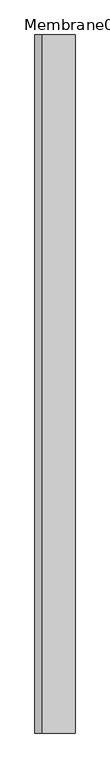
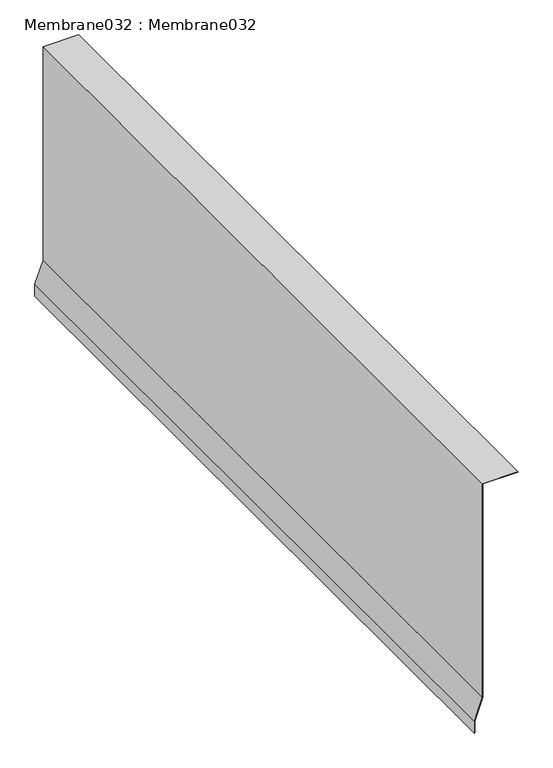
"""IFC4 building model written with IfcOpenShell, lengths in millimetres: proxy geometry, Membrane032 : Membrane032."""

from ifc_helpers import new_model, si_unit, frame, origin, place, context, project, spatial, polyline, outline, extrude, source, transform, mapped, element, save


def membrane032_membrane032_113c58a5(model_context):
    return source(origin(), model_context, "Body", "SweptSolid", [
        extrude(outline(polyline([(40237.828125, -2674.0896171), (40237.828125, -2767.6617221), (39645.0411306, -2767.6617221), (39585.9385394, -2789.1733061), (39552.6918208, -2789.1733061), (39552.6918208, -2788.1733061), (39585.7622124, -2788.1733061), (39644.8648036, -2766.6617221), (40236.828125, -2766.6617221), (40236.828125, -2674.0896171), (40237.828125, -2674.0896171)])), frame((0.0, -1052.8906574, 0.0), z_axis=(0.0, 1.0, 0.0), x_axis=(0.0, 0.0, 1.0)), (0.0, 0.0, 1.0), 2000.0),
    ])


if __name__ == "__main__":
    model = new_model("IFC4")
    model_context = context("Model", 3, world=origin())
    ifc_project = project(units=[si_unit("LENGTHUNIT", "METRE", prefix="MILLI")], contexts=[model_context])
    site = spatial("IfcSite", under=ifc_project)
    building = spatial("IfcBuilding", under=site)
    placement = place(None, origin())
    membrane032_membrane032_shape = membrane032_membrane032_113c58a5(model_context)
    element("IfcBuildingElementProxy", 1, Name="Membrane032 : Membrane032", ObjectType="Membrane032 : Membrane032", at=placement, inside=building, context=model_context, shape_type="MappedRepresentation", body=[
        mapped(membrane032_membrane032_shape, transform((0.0, 0.0, 0.0), x_axis=(1.0, 0.0, 0.0), y_axis=(0.0, 1.0, 0.0), z_axis=(0.0, 0.0, 1.0))),
    ])
    save(model, "model.ifc")

# Revit data of these elements
# Type "Membrane032 : Membrane032"
#   NameOverride = "Membrane032"
# Element 1 (IfcBuildingElementProxy, "Membrane032 : Membrane032")
#   Materials on its faces: "(2) LAYERS OF ICE & WATER SHIELD (BITUTHANE) UNDER STUCCO"
# Materials
#   "(2) LAYERS OF ICE & WATER SHIELD (BITUTHANE) UNDER STUCCO": class "Unassigned", colour RGB 186 255 159, transparency 0, Cost = 0
